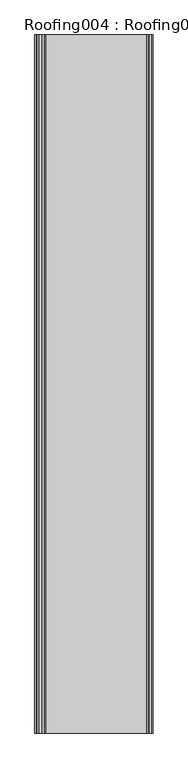
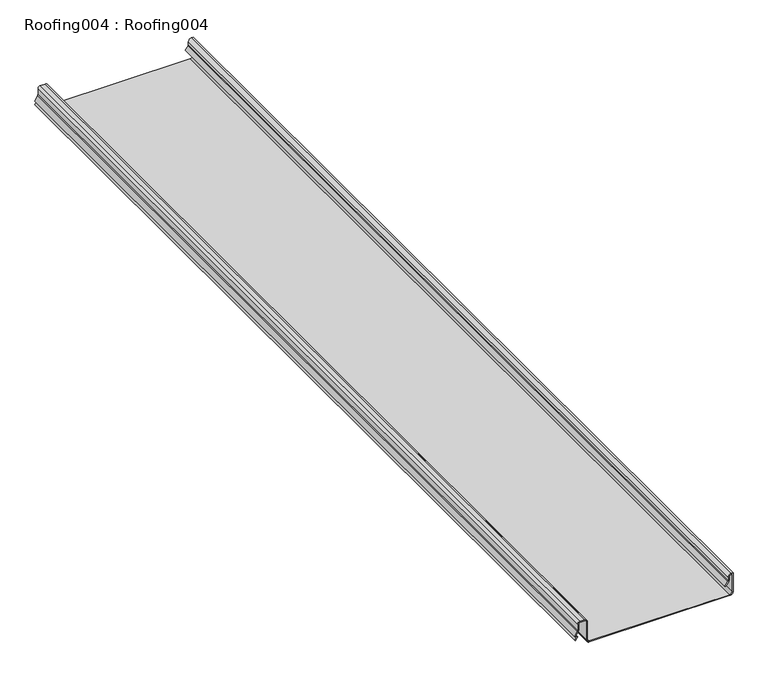
"""IFC4 building model written with IfcOpenShell, lengths in millimetres: proxy geometry, Roofing004 : Roofing004."""

from ifc_helpers import new_model, si_unit, point, frame, frame_2d, origin, place, context, project, spatial, polyline, circle_curve, trimmed, segment, composite_curve, outline, extrude, source, transform, mapped, element, save


def roofing004_roofing004_1c7537e7(model_context):
    return source(origin(), model_context, "Body", "SweptSolid", [
        extrude(outline(composite_curve([segment(trimmed(circle_curve(frame_2d((42567.7361552, -1807.009115)), 5.08), [point((42564.7531257, -1802.8971891))], [point((42567.7361552, -1801.929115))], False, "CARTESIAN"), True, "CONTINUOUS"), segment(polyline([(42567.7361552, -1801.929115), (42574.4927135, -1801.929115)]), True, "CONTINUOUS"), segment(trimmed(circle_curve(frame_2d((42574.4927135, -1796.849115)), 5.08), [point((42574.4927135, -1801.929115))], [point((42579.5727135, -1796.849115))], True, "CARTESIAN"), True, "CONTINUOUS"), segment(polyline([(42579.5727135, -1796.849115), (42579.5727135, -1795.2543103), (42539.835526, -1795.2543103)]), True, "CONTINUOUS"), segment(trimmed(circle_curve(frame_2d((42539.835526, -1800.3343103)), 5.08), [point((42539.835526, -1795.2543103))], [point((42534.755526, -1800.3343103))], True, "CARTESIAN"), True, "CONTINUOUS"), segment(polyline([(42534.755526, -1800.3343103), (42534.755526, -2100.6083924)]), True, "CONTINUOUS"), segment(trimmed(circle_curve(frame_2d((42539.835526, -2100.6083924)), 5.08), [point((42534.755526, -2100.6083924))], [point((42539.835526, -2105.6883924))], True, "CARTESIAN"), True, "CONTINUOUS"), segment(polyline([(42539.835526, -2105.6883924), (42581.4489635, -2105.6883924)]), True, "CONTINUOUS"), segment(trimmed(circle_curve(frame_2d((42581.4489635, -2110.7683924)), 5.08), [point((42581.4489635, -2105.6883924))], [point((42586.5289635, -2110.7683924))], False, "CARTESIAN"), True, "CONTINUOUS"), segment(polyline([(42586.5289635, -2110.7683924), (42586.5289635, -2120.7761693)]), True, "CONTINUOUS"), segment(trimmed(circle_curve(frame_2d((42581.4489635, -2120.7761693)), 5.08), [point((42586.5289635, -2120.7761693))], [point((42581.4489635, -2125.8561693))], False, "CARTESIAN"), True, "CONTINUOUS"), segment(polyline([(42581.4489635, -2125.8561693), (42568.2663894, -2125.8561693)]), True, "CONTINUOUS"), segment(trimmed(circle_curve(frame_2d((42568.2663894, -2130.9361693)), 5.08), [point((42568.2663894, -2125.8561693))], [point((42565.7623779, -2126.5161776))], True, "CARTESIAN"), True, "CONTINUOUS"), segment(polyline([(42565.7623779, -2126.5161776), (42555.2047448, -2132.4972825), (42552.7633385, -2128.33322), (42547.161776, -2132.3322435), (42545.9997023, -2130.704489), (42553.3820175, -2125.4341646), (42555.9334157, -2129.7858294), (42564.7765466, -2124.7760233)]), True, "CONTINUOUS"), segment(trimmed(circle_curve(frame_2d((42568.2663894, -2130.9361693)), 7.08), [point((42564.7765466, -2124.7760233))], [point((42568.2663894, -2123.8561693))], False, "CARTESIAN"), True, "CONTINUOUS"), segment(polyline([(42568.2663894, -2123.8561693), (42581.4489635, -2123.8561693)]), True, "CONTINUOUS"), segment(trimmed(circle_curve(frame_2d((42581.4489635, -2120.7761693)), 3.08), [point((42581.4489635, -2123.8561693))], [point((42584.5289635, -2120.7761693))], True, "CARTESIAN"), True, "CONTINUOUS"), segment(polyline([(42584.5289635, -2120.7761693), (42584.5289635, -2110.7683924)]), True, "CONTINUOUS"), segment(trimmed(circle_curve(frame_2d((42581.4489635, -2110.7683924)), 3.08), [point((42584.5289635, -2110.7683924))], [point((42581.4489635, -2107.6883924))], True, "CARTESIAN"), True, "CONTINUOUS"), segment(polyline([(42581.4489635, -2107.6883924), (42539.835526, -2107.6883924)]), True, "CONTINUOUS"), segment(trimmed(circle_curve(frame_2d((42539.835526, -2100.6083924)), 7.08), [point((42539.835526, -2107.6883924))], [point((42532.755526, -2100.6083924))], False, "CARTESIAN"), True, "CONTINUOUS"), segment(polyline([(42532.755526, -2100.6083924), (42532.755526, -1800.3343103)]), True, "CONTINUOUS"), segment(trimmed(circle_curve(frame_2d((42539.835526, -1800.3343103)), 7.08), [point((42532.755526, -1800.3343103))], [point((42539.835526, -1793.2543103))], False, "CARTESIAN"), True, "CONTINUOUS"), segment(polyline([(42539.835526, -1793.2543103), (42581.5727135, -1793.2543103), (42581.5727135, -1796.849115)]), True, "CONTINUOUS"), segment(trimmed(circle_curve(frame_2d((42574.4927135, -1796.849115)), 7.08), [point((42581.5727135, -1796.849115))], [point((42574.4927135, -1803.929115))], False, "CARTESIAN"), True, "CONTINUOUS"), segment(polyline([(42574.4927135, -1803.929115), (42567.7361552, -1803.929115)]), True, "CONTINUOUS"), segment(trimmed(circle_curve(frame_2d((42567.7361552, -1807.009115)), 3.08), [point((42567.7361552, -1803.929115))], [point((42565.9275467, -1804.5160576))], True, "CARTESIAN"), True, "CONTINUOUS"), segment(polyline([(42565.9275467, -1804.5160576), (42557.4533846, -1810.6637061), (42556.2789635, -1809.0448377), (42564.7531257, -1802.8971891)]), True, "CONTINUOUS")], self_intersect=False)), frame((0.0, -1052.8906574, 0.0), z_axis=(0.0, 1.0, 0.0), x_axis=(0.0, 0.0, 1.0)), (0.0, 0.0, 1.0), 2000.0),
    ])


if __name__ == "__main__":
    model = new_model("IFC4")
    model_context = context("Model", 3, world=origin())
    ifc_project = project(units=[si_unit("LENGTHUNIT", "METRE", prefix="MILLI")], contexts=[model_context])
    site = spatial("IfcSite", under=ifc_project)
    building = spatial("IfcBuilding", under=site)
    placement = place(None, origin())
    roofing004_roofing004_shape = roofing004_roofing004_1c7537e7(model_context)
    element("IfcBuildingElementProxy", 1, Name="Roofing004 : Roofing004", ObjectType="Roofing004 : Roofing004", at=placement, inside=building, context=model_context, shape_type="MappedRepresentation", body=[
        mapped(roofing004_roofing004_shape, transform((0.0, 0.0, 0.0), x_axis=(1.0, 0.0, 0.0), y_axis=(0.0, 1.0, 0.0), z_axis=(0.0, 0.0, 1.0))),
    ])
    save(model, "model.ifc")

# Revit data of these elements
# Type "Roofing004 : Roofing004"
#   NameOverride = "Roofing004"
# Element 1 (IfcBuildingElementProxy, "Roofing004 : Roofing004")
#   Materials on its faces: "STANDING SEAM METAL ROOF"
# Materials
#   "STANDING SEAM METAL ROOF": class "Unassigned", colour RGB 128 128 128, transparency 0
